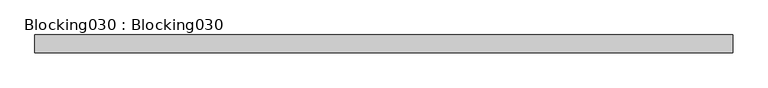
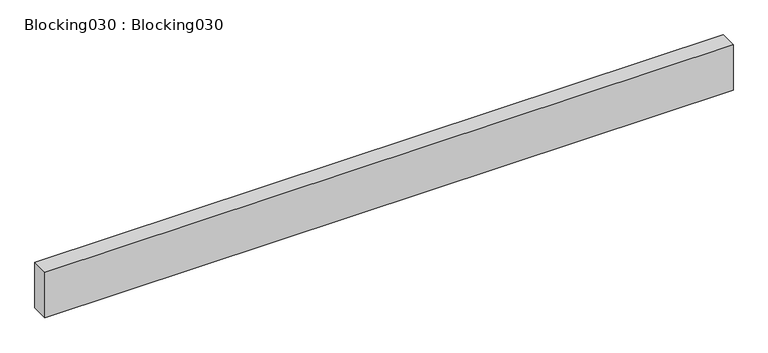
"""IFC4 building model written with IfcOpenShell, lengths in millimetres: proxy geometry, Blocking030 : Blocking030."""

from ifc_helpers import new_model, si_unit, frame, origin, place, context, project, spatial, polyline, outline, extrude, source, transform, mapped, element, save


def blocking030_blocking030_0ec92764(model_context):
    return source(origin(), model_context, "Body", "SweptSolid", [
        extrude(outline(polyline([(14383.0178845, -4497.8425368), (14383.0178845, -4548.6425368), (12383.0178845, -4548.6425368), (12383.0178845, -4497.8425368), (14383.0178845, -4497.8425368)])), frame((0.0, 0.0, 39019.0959974), z_axis=(0.0, 0.0, 1.0), x_axis=(1.0, 0.0, 0.0)), (0.0, 0.0, 1.0), 139.7),
    ])


if __name__ == "__main__":
    model = new_model("IFC4")
    model_context = context("Model", 3, world=origin())
    ifc_project = project(units=[si_unit("LENGTHUNIT", "METRE", prefix="MILLI")], contexts=[model_context])
    site = spatial("IfcSite", under=ifc_project)
    building = spatial("IfcBuilding", under=site)
    placement = place(None, origin())
    blocking030_blocking030_shape = blocking030_blocking030_0ec92764(model_context)
    element("IfcBuildingElementProxy", 1, Name="Blocking030 : Blocking030", ObjectType="Blocking030 : Blocking030", at=placement, inside=building, context=model_context, shape_type="MappedRepresentation", body=[
        mapped(blocking030_blocking030_shape, transform((0.0, 0.0, 0.0), x_axis=(1.0, 0.0, 0.0), y_axis=(0.0, 1.0, 0.0), z_axis=(0.0, 0.0, 1.0))),
    ])
    save(model, "model.ifc")

# Revit data of these elements
# Type "Blocking030 : Blocking030"
#   NameOverride = "Blocking030"
# Element 1 (IfcBuildingElementProxy, "Blocking030 : Blocking030")
#   Materials on its faces: "WOOD BLOCKING AS REQUIRED"
# Materials
#   "WOOD BLOCKING AS REQUIRED": class "Unassigned", colour RGB 166 124 85, transparency 0, Cost = 0
